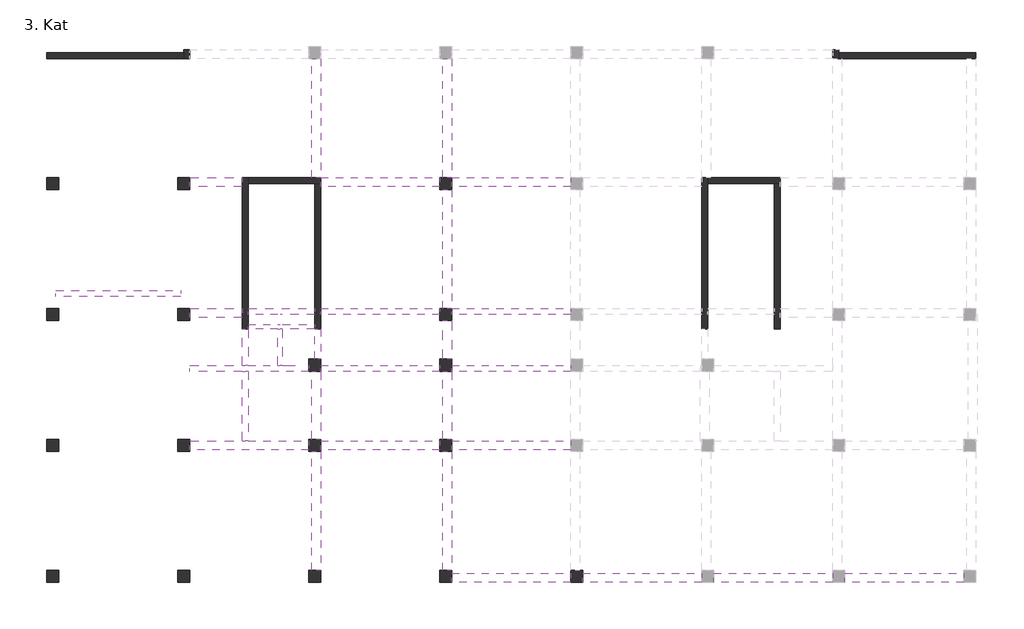
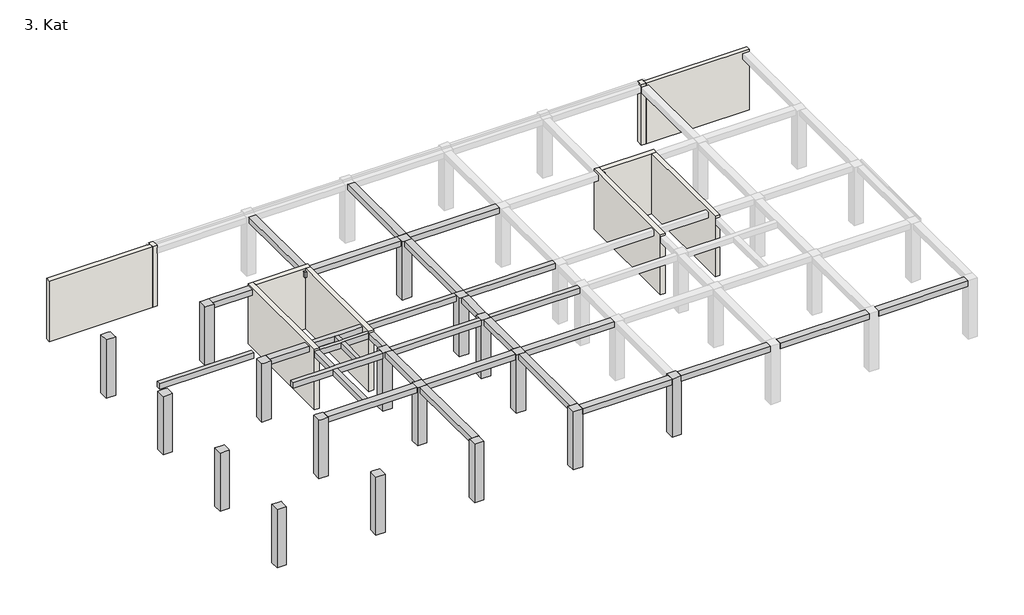
# One storey, part 1 of 2: 31 beams, 17 columns, 10 walls.
"""IFC4 building model written with IfcOpenShell, lengths in millimetres."""

from ifc_helpers import new_model, si_unit, frame, origin, place, context, project, spatial, polyline, outline, extrude, faceted_brep, element, save

model = new_model("IFC4")

# Units and contexts
model_context = context("Model", 3, world=origin())
ifc_project = project(units=[si_unit("LENGTHUNIT", "METRE", prefix="MILLI")], contexts=[model_context])

# Site, building, storey
site = spatial("IfcSite", under=ifc_project)
building = spatial("IfcBuilding", under=site)
storey = spatial("IfcBuildingStorey", under=building, Name="3. Kat", Elevation=15500.0)

# Beams
placement = place(None, origin())
element("IfcBeam", 1, ObjectType="M_Concrete-Rectangular Beam : 40x70cm kiriş 2", at=placement, inside=storey, context=model_context, shape_type="SweptSolid", body=[
    extrude(outline(polyline([(204.0222331, 18150.0006424), (204.0222331, 18550.0006424), (8299.9996735, 18550.0006424), (8299.9996735, 18150.0006424), (204.0222331, 18150.0006424)])), frame((0.0, 0.0, 20300.0), z_axis=(0.0, 0.0, 1.0), x_axis=(1.0, 0.0, 0.0)), (0.0, 0.0, 1.0), 500.0),
])
element("IfcBeam", 2, ObjectType="M_Concrete-Rectangular Beam : 60x70cm kiriş", at=placement, inside=storey, context=model_context, shape_type="SweptSolid", body=[
    extrude(outline(polyline([(16799.9996817, 33600.0009197), (17399.9996817, 33600.0009197), (17399.9996817, 25900.0003816), (16799.9996817, 25900.0003816), (16799.9996817, 33600.0009197)])), frame((0.0, 0.0, 20300.0), z_axis=(0.0, 0.0, 1.0), x_axis=(1.0, 0.0, 0.0)), (0.0, 0.0, 1.0), 500.0),
])
element("IfcBeam", 3, ObjectType="M_Concrete-Rectangular Beam : 60x70cm kiriş", at=placement, inside=storey, context=model_context, shape_type="SweptSolid", body=[
    extrude(outline(polyline([(25899.9996503, 25900.0004105), (25299.9996503, 25900.0004105), (25299.9996503, 33600.0009197), (25899.9996503, 33600.0009197), (25899.9996503, 25900.0004105)])), frame((0.0, 0.0, 20300.0), z_axis=(0.0, 0.0, 1.0), x_axis=(1.0, 0.0, 0.0)), (0.0, 0.0, 1.0), 500.0),
])
element("IfcBeam", 4, ObjectType="M_Concrete-Rectangular Beam : 60x70cm kiriş", at=placement, inside=storey, context=model_context, shape_type="Brep", body=[
    faceted_brep([(25099.9993907, 25900.0000279, 20300.0), (17399.9996817, 25900.0000279, 20300.0), (17399.9996817, 25900.0000279, 20800.0), (25099.9993907, 25900.0000279, 20800.0), (17399.9995362, 25300.0000279, 20300.0), (25099.9993907, 25300.0000279, 20300.0), (25099.9993907, 25300.0000279, 20800.0), (17399.9995362, 25300.0000279, 20800.0)], [[[0, 1, 2, 3]], [[4, 1, 0, 5]], [[5, 6, 7, 4]], [[4, 7, 2, 1]], [[3, 2, 7, 6]], [[5, 0, 3, 6]]]),
    faceted_brep([(16799.9996817, 25500.0003816, 20300.0), (16799.9996817, 25300.0000279, 20300.0), (16799.9996817, 25300.0000279, 20800.0), (16799.9996817, 25500.0003816, 20800.0), (16999.9995362, 25500.0003816, 20800.0), (16999.9995362, 25500.0003816, 20300.0), (16999.9995362, 25300.0000279, 20300.0), (16999.9995362, 25300.0000279, 20800.0)], [[[0, 1, 2, 3]], [[0, 3, 4, 5]], [[6, 5, 4, 7]], [[1, 0, 5, 6]], [[2, 1, 6, 7]], [[3, 2, 7, 4]]]),
])
element("IfcBeam", 5, ObjectType="M_Concrete-Rectangular Beam : 60x70cm kiriş", at=placement, inside=storey, context=model_context, shape_type="SweptSolid", body=[
    extrude(outline(polyline([(8899.9993907, 25299.9999925), (8899.9993907, 25899.9999925), (12300.0064017, 25899.9999925), (12300.0064017, 25299.9999925), (8899.9993907, 25299.9999925)])), frame((0.0, 0.0, 20300.0), z_axis=(0.0, 0.0, 1.0), x_axis=(1.0, 0.0, 0.0)), (0.0, 0.0, 1.0), 500.0),
])
element("IfcBeam", 6, ObjectType="M_Concrete-Rectangular Beam : 60x70cm kiriş", at=placement, inside=storey, context=model_context, shape_type="Brep", body=[
    faceted_brep([(8899.9993907, 16800.0003643, 20800.0), (8899.9993907, 16800.0003643, 20300.0), (12300.0064017, 16800.0003643, 20300.0), (12300.0064017, 16800.0003643, 20800.0), (8899.9996735, 17400.0003643, 20300.0), (12300.0064017, 17400.0003643, 20300.0), (8899.9996735, 17400.0003643, 20800.0), (12300.0064017, 17400.0003643, 20800.0)], [[[0, 1, 2, 3]], [[1, 4, 5, 2]], [[4, 6, 7, 5]], [[6, 4, 1, 0]], [[6, 0, 3, 7]], [[3, 2, 5, 7]]]),
])
element("IfcBeam", 7, ObjectType="M_Concrete-Rectangular Beam : 40x70cm kiriş 2", at=placement, inside=storey, context=model_context, shape_type="Brep", body=[
    faceted_brep([(12700.0064017, 17000.0003638, 20800.0), (12700.0064017, 17000.0003638, 20300.0), (14600.0010318, 17000.0003638, 20300.0), (14900.0010318, 17000.0003638, 20300.0), (16999.9995362, 17000.0003638, 20300.0), (16999.9995362, 17000.0003638, 20800.0), (14900.0010318, 17000.0003638, 20800.0), (14600.0010318, 17000.0003638, 20800.0), (12700.0064017, 17400.0003638, 20300.0), (16999.9995362, 17400.0003638, 20300.0), (12700.0064017, 17400.0003638, 20800.0), (16999.9995362, 17400.0003638, 20800.0)], [[[0, 1, 2, 3, 4, 5, 6, 7]], [[1, 8, 9, 4, 3, 2]], [[8, 10, 11, 9]], [[8, 1, 0, 10]], [[10, 0, 7, 6, 5, 11]], [[5, 4, 9, 11]]]),
])
element("IfcBeam", 8, ObjectType="M_Concrete-Rectangular Beam : 40x70cm kiriş 2", at=placement, inside=storey, context=model_context, shape_type="SweptSolid", body=[
    extrude(outline(polyline([(17399.9995362, 17400.0003766), (25099.999715, 17400.0003766), (25099.999715, 17000.0003766), (17399.9995362, 17000.0003766), (17399.9995362, 17400.0003766)])), frame((0.0, 0.0, 20300.0), z_axis=(0.0, 0.0, 1.0), x_axis=(1.0, 0.0, 0.0)), (0.0, 0.0, 1.0), 500.0),
])
element("IfcBeam", 9, ObjectType="M_Concrete-Rectangular Beam : 40x70cm kiriş 2", at=placement, inside=storey, context=model_context, shape_type="Brep", body=[
    faceted_brep([(16599.9993867, 13700.0003638, 20300.0), (14900.0010318, 13700.0003638, 20300.0), (14600.0010318, 13700.0003638, 20300.0), (12700.0064017, 13700.0003638, 20300.0), (12300.0064017, 13700.0003638, 20300.0), (8899.9996095, 13700.0003638, 20300.0), (8899.9996095, 13700.0003638, 20800.0), (12300.0064017, 13700.0003638, 20800.0), (12700.0064017, 13700.0003638, 20800.0), (14600.0010318, 13700.0003638, 20800.0), (14900.0010318, 13700.0003638, 20800.0), (16599.9993867, 13700.0003638, 20800.0), (16599.9993867, 13300.0003638, 20300.0), (12700.0064017, 13300.0003638, 20300.0), (12300.0064017, 13300.0003638, 20300.0), (8899.9996095, 13300.0003638, 20300.0), (16599.9993867, 13300.0003638, 20800.0), (12700.0064017, 13300.0003638, 20800.0), (12300.0064017, 13300.0003638, 20800.0), (8899.9996095, 13300.0003638, 20800.0)], [[[0, 1, 2, 3, 4, 5, 6, 7, 8, 9, 10, 11]], [[5, 4, 3, 2, 1, 0, 12, 13, 14, 15]], [[15, 14, 13, 12, 16, 17, 18, 19]], [[5, 15, 19, 6]], [[11, 10, 9, 8, 7, 6, 19, 18, 17, 16]], [[12, 0, 11, 16]]]),
])
element("IfcBeam", 10, ObjectType="M_Concrete-Rectangular Beam : 40x70cm kiriş 2", at=placement, inside=storey, context=model_context, shape_type="SweptSolid", body=[
    extrude(outline(polyline([(12700.0064017, 13700.0003638), (12300.0064017, 13700.0003638), (12300.0064017, 16050.000156), (12700.0064017, 16050.000156), (12700.0064017, 13700.0003638)])), frame((0.0, 0.0, 20300.0), z_axis=(0.0, 0.0, 1.0), x_axis=(1.0, 0.0, 0.0)), (0.0, 0.0, 1.0), 500.0),
])
element("IfcBeam", 11, ObjectType="M_Concrete-Rectangular Beam : 40x70cm kiriş 2", at=placement, inside=storey, context=model_context, shape_type="SweptSolid", body=[
    extrude(outline(polyline([(17399.9995362, 14099.9451047), (16999.9995362, 14099.9451047), (16999.9995362, 16050.0003816), (17399.9995362, 16050.0003816), (17399.9995362, 14099.9451047)])), frame((0.0, 0.0, 20300.0), z_axis=(0.0, 0.0, 1.0), x_axis=(1.0, 0.0, 0.0)), (0.0, 0.0, 1.0), 500.0),
])
element("IfcBeam", 12, ObjectType="M_Concrete-Rectangular Beam : 30x70cm kiriş 3", at=placement, inside=storey, context=model_context, shape_type="Brep", body=[
    faceted_brep([(12700.0064017, 16350.0003638, 20300.0), (12700.0064017, 16350.0003638, 20800.0), (14600.0010318, 16350.0003638, 20800.0), (14900.0010318, 16350.0003638, 20800.0), (16999.9995362, 16350.0003638, 20800.0), (16999.9995362, 16350.0003638, 20300.0), (14900.0010318, 16350.0003638, 20300.0), (14600.0010318, 16350.0003638, 20300.0), (16999.9995362, 16050.0003638, 20300.0), (14900.0010318, 16050.0003638, 20300.0), (14600.0010318, 16050.0003638, 20300.0), (12700.0064017, 16050.0003638, 20300.0), (16999.9995362, 16050.0003638, 20800.0), (14900.0010318, 16050.0003638, 20800.0), (14600.0010318, 16050.0003638, 20800.0), (12700.0064017, 16050.0003638, 20800.0)], [[[0, 1, 2, 3, 4, 5, 6, 7]], [[5, 8, 9, 10, 11, 0, 7, 6]], [[11, 10, 9, 8, 12, 13, 14, 15]], [[11, 15, 1, 0]], [[5, 4, 12, 8]], [[15, 14, 13, 12, 4, 3, 2, 1]]]),
])
element("IfcBeam", 13, ObjectType="M_Concrete-Rectangular Beam : 30x70cm kiriş 3", at=placement, inside=storey, context=model_context, shape_type="SweptSolid", body=[
    extrude(outline(polyline([(14900.0010318, 13700.0003638), (14600.0010318, 13700.0003638), (14600.0010318, 16050.0003638), (14900.0010318, 16050.0003638), (14900.0010318, 13700.0003638)])), frame((0.0, 0.0, 20300.0), z_axis=(0.0, 0.0, 1.0), x_axis=(1.0, 0.0, 0.0)), (0.0, 0.0, 1.0), 500.0),
    extrude(outline(polyline([(14600.0010318, 17000.0003638), (14900.0010318, 17000.0003638), (14900.0010318, 16350.0003638), (14600.0010318, 16350.0003638), (14600.0010318, 17000.0003638)])), frame((0.0, 0.0, 20300.0), z_axis=(0.0, 0.0, 1.0), x_axis=(1.0, 0.0, 0.0)), (0.0, 0.0, 1.0), 500.0),
])
element("IfcBeam", 14, ObjectType="M_Concrete-Rectangular Beam : 60x70cm kiriş", at=placement, inside=storey, context=model_context, shape_type="Brep", body=[
    faceted_brep([(8899.9993907, 8200.0009197, 20300.0), (16599.9993907, 8200.0009197, 20300.0), (16599.9993907, 8200.0009197, 20800.0), (8899.9993907, 8200.0009197, 20800.0), (8899.9993907, 8800.0009197, 20300.0), (12300.0064017, 8800.0009197, 20300.0), (12700.0064017, 8800.0009197, 20300.0), (16599.9993907, 8800.0009197, 20300.0), (8899.9993907, 8800.0009197, 20800.0), (12300.0064017, 8800.0009197, 20800.0), (12700.0064017, 8800.0009197, 20800.0), (16599.9993907, 8800.0009197, 20800.0)], [[[0, 1, 2, 3]], [[1, 0, 4, 5, 6, 7]], [[7, 6, 5, 4, 8, 9, 10, 11]], [[3, 2, 11, 10, 9, 8]], [[4, 0, 3, 8]], [[1, 7, 11, 2]]]),
])
element("IfcBeam", 15, ObjectType="M_Concrete-Rectangular Beam : 60x70cm kiriş", at=placement, inside=storey, context=model_context, shape_type="SweptSolid", body=[
    extrude(outline(polyline([(17399.9997293, 8900.0009197), (16799.9997293, 8900.0009197), (16799.9997293, 13299.9451047), (17399.9997293, 13299.9451047), (17399.9997293, 8900.0009197)])), frame((0.0, 0.0, 20300.0), z_axis=(0.0, 0.0, 1.0), x_axis=(1.0, 0.0, 0.0)), (0.0, 0.0, 1.0), 500.0),
])
element("IfcBeam", 16, ObjectType="M_Concrete-Rectangular Beam : 60x70cm kiriş", at=placement, inside=storey, context=model_context, shape_type="SweptSolid", body=[
    extrude(outline(polyline([(16799.9997451, 400.0009197), (16799.9997451, 8099.9999409), (17399.9997451, 8099.9999409), (17399.9997451, 400.0009197), (16799.9997451, 400.0009197)])), frame((0.0, 0.0, 20300.0), z_axis=(0.0, 0.0, 1.0), x_axis=(1.0, 0.0, 0.0)), (0.0, 0.0, 1.0), 500.0),
])
element("IfcBeam", 17, ObjectType="M_Concrete-Rectangular Beam : 40x70cm kiriş 2", at=placement, inside=storey, context=model_context, shape_type="SweptSolid", body=[
    extrude(outline(polyline([(12300.0064017, 13300.0003638), (12700.0064017, 13300.0003638), (12700.0064017, 8800.0009197), (12300.0064017, 8800.0009197), (12300.0064017, 13300.0003638)])), frame((0.0, 0.0, 20300.0), z_axis=(0.0, 0.0, 1.0), x_axis=(1.0, 0.0, 0.0)), (0.0, 0.0, 1.0), 500.0),
])
element("IfcBeam", 18, ObjectType="M_Concrete-Rectangular Beam : 60x70cm kiriş", at=placement, inside=storey, context=model_context, shape_type="SweptSolid", body=[
    extrude(outline(polyline([(25299.9997233, 400.0009197), (25299.9997233, 8100.0009197), (25899.9997233, 8100.0009197), (25899.9997233, 400.0009197), (25299.9997233, 400.0009197)])), frame((0.0, 0.0, 20300.0), z_axis=(0.0, 0.0, 1.0), x_axis=(1.0, 0.0, 0.0)), (0.0, 0.0, 1.0), 500.0),
])
element("IfcBeam", 19, ObjectType="M_Concrete-Rectangular Beam : 60x70cm kiriş", at=placement, inside=storey, context=model_context, shape_type="SweptSolid", body=[
    extrude(outline(polyline([(25099.9993907, 8200.0009197), (17399.9993907, 8200.0009197), (17399.9993907, 8800.0009197), (25099.9993907, 8800.0009197), (25099.9993907, 8200.0009197)])), frame((0.0, 0.0, 20300.0), z_axis=(0.0, 0.0, 1.0), x_axis=(1.0, 0.0, 0.0)), (0.0, 0.0, 1.0), 500.0),
])
element("IfcBeam", 20, ObjectType="M_Concrete-Rectangular Beam : 60x70cm kiriş", at=placement, inside=storey, context=model_context, shape_type="SweptSolid", body=[
    extrude(outline(polyline([(25899.9997233, 8900.0009197), (25299.9997233, 8900.0009197), (25299.9997233, 13300.0003995), (25899.9997233, 13300.0003995), (25899.9997233, 8900.0009197)])), frame((0.0, 0.0, 20300.0), z_axis=(0.0, 0.0, 1.0), x_axis=(1.0, 0.0, 0.0)), (0.0, 0.0, 1.0), 500.0),
])
element("IfcBeam", 21, ObjectType="M_Concrete-Rectangular Beam : 40x70cm kiriş 2", at=placement, inside=storey, context=model_context, shape_type="Brep", body=[
    faceted_brep([(25099.9997415, 13700.0003995, 20800.0), (25099.9997415, 13700.0003995, 20300.0), (17399.9993907, 13700.0003995, 20300.0), (17399.9993907, 13700.0003995, 20800.0), (17399.9997293, 13300.0003995, 20300.0), (25099.9997415, 13300.0003995, 20300.0), (17399.9997293, 13300.0003995, 20800.0), (25099.9997415, 13300.0003995, 20800.0)], [[[0, 1, 2, 3]], [[4, 2, 1, 5]], [[6, 4, 5, 7]], [[4, 6, 3, 2]], [[3, 6, 7, 0]], [[5, 1, 0, 7]]]),
])
element("IfcBeam", 22, ObjectType="M_Concrete-Rectangular Beam : 60x70cm kiriş", at=placement, inside=storey, context=model_context, shape_type="SweptSolid", body=[
    extrude(outline(polyline([(25299.9997233, 14100.0003995), (25299.9997233, 16600.0009197), (25899.9997233, 16600.0009197), (25899.9997233, 14100.0003995), (25299.9997233, 14100.0003995)])), frame((0.0, 0.0, 20300.0), z_axis=(0.0, 0.0, 1.0), x_axis=(1.0, 0.0, 0.0)), (0.0, 0.0, 1.0), 500.0),
])
element("IfcBeam", 23, ObjectType="M_Concrete-Rectangular Beam : 60x70cm kiriş", at=placement, inside=storey, context=model_context, shape_type="SweptSolid", body=[
    extrude(outline(polyline([(25299.999682, 25099.9999518), (25899.999682, 25099.9999518), (25899.999682, 17400.0009197), (25299.999682, 17400.0009197), (25299.999682, 25099.9999518)])), frame((0.0, 0.0, 20300.0), z_axis=(0.0, 0.0, 1.0), x_axis=(1.0, 0.0, 0.0)), (0.0, 0.0, 1.0), 500.0),
])
element("IfcBeam", 24, ObjectType="M_Concrete-Rectangular Beam : 60x70cm kiriş", at=placement, inside=storey, context=model_context, shape_type="Brep", body=[
    faceted_brep([(25899.9996503, 25900.0003995, 20300.0), (25899.9996503, 25900.0003995, 20800.0), (33599.9993907, 25900.0003995, 20800.0), (33599.9993907, 25900.0003995, 20300.0), (25899.9993907, 25300.0003995, 20300.0), (33599.9993907, 25300.0003995, 20300.0), (25899.9993907, 25300.0003995, 20800.0), (33599.9993907, 25300.0003995, 20800.0)], [[[0, 1, 2, 3]], [[4, 0, 3, 5]], [[6, 4, 5, 7]], [[1, 0, 4, 6]], [[1, 6, 7, 2]], [[3, 2, 7, 5]]]),
])
element("IfcBeam", 25, ObjectType="M_Concrete-Rectangular Beam : 40x70cm kiriş 2", at=placement, inside=storey, context=model_context, shape_type="Brep", body=[
    faceted_brep([(33599.9993907, 17000.0007711, 20300.0), (33599.9993907, 17000.0007711, 20800.0), (25899.9993907, 17000.0007711, 20800.0), (25899.9993907, 17000.0007711, 20300.0), (25899.999682, 17400.0007711, 20300.0), (33599.9994953, 17400.0007711, 20300.0), (25899.999682, 17400.0007711, 20800.0), (33599.9994953, 17400.0007711, 20800.0)], [[[0, 1, 2, 3]], [[3, 4, 5, 0]], [[4, 6, 7, 5]], [[3, 2, 6, 4]], [[5, 7, 1, 0]], [[7, 6, 2, 1]]]),
])
element("IfcBeam", 26, ObjectType="M_Concrete-Rectangular Beam : 40x70cm kiriş 2", at=placement, inside=storey, context=model_context, shape_type="Brep", body=[
    faceted_brep([(25899.9997233, 13300.0003995, 20800.0), (25899.9997233, 13300.0003995, 20300.0), (33599.9993907, 13300.0003995, 20300.0), (33599.9993907, 13300.0003995, 20800.0), (25899.9993907, 13700.0003995, 20300.0), (33599.9993907, 13700.0003995, 20300.0), (33599.9993907, 13700.0003995, 20800.0), (25899.9993907, 13700.0003995, 20800.0)], [[[0, 1, 2, 3]], [[1, 4, 5, 2]], [[6, 5, 4, 7]], [[1, 0, 7, 4]], [[7, 0, 3, 6]], [[3, 2, 5, 6]]]),
])
element("IfcBeam", 27, ObjectType="M_Concrete-Rectangular Beam : 60x70cm kiriş", at=placement, inside=storey, context=model_context, shape_type="Brep", body=[
    faceted_brep([(25899.9993907, 8200.0009197, 20800.0), (25899.9993907, 8200.0009197, 20300.0), (33599.9993907, 8200.0009197, 20300.0), (33599.9993907, 8200.0009197, 20800.0), (33599.9994953, 8800.0009197, 20300.0), (25899.9993907, 8800.0009197, 20300.0), (33599.9994953, 8800.0009197, 20800.0), (25899.9993907, 8800.0009197, 20800.0)], [[[0, 1, 2, 3]], [[4, 2, 1, 5]], [[6, 4, 5, 7]], [[4, 6, 3, 2]], [[3, 6, 7, 0]], [[1, 0, 7, 5]]]),
])
element("IfcBeam", 28, ObjectType="M_Concrete-Rectangular Beam : 60x70cm kiriş", at=placement, inside=storey, context=model_context, shape_type="Brep", body=[
    faceted_brep([(34399.9993907, -399.9996882, 20800.0), (34399.9993907, -399.9996882, 20300.0), (42099.9993899, -399.9996882, 20300.0), (42099.9993899, -399.9996882, 20800.0), (42099.999723, 200.0003118, 20300.0), (34399.9993907, 200.0003118, 20300.0), (42099.999723, 200.0003118, 20800.0), (34399.9993907, 200.0003118, 20800.0)], [[[0, 1, 2, 3]], [[4, 2, 1, 5]], [[6, 4, 5, 7]], [[4, 6, 3, 2]], [[3, 6, 7, 0]], [[1, 0, 7, 5]]]),
])
element("IfcBeam", 29, ObjectType="M_Concrete-Rectangular Beam : 60x70cm kiriş", at=placement, inside=storey, context=model_context, shape_type="SweptSolid", body=[
    extrude(outline(polyline([(25899.9993907, -399.9996882), (25899.9993907, 200.0003118), (33599.9993907, 200.0003118), (33599.9993907, -399.9996882), (25899.9993907, -399.9996882)])), frame((0.0, 0.0, 20300.0), z_axis=(0.0, 0.0, 1.0), x_axis=(1.0, 0.0, 0.0)), (0.0, 0.0, 1.0), 500.0),
])
element("IfcBeam", 30, ObjectType="M_Concrete-Rectangular Beam : 60x70cm kiriş", at=placement, inside=storey, context=model_context, shape_type="Brep", body=[
    faceted_brep([(42899.9997771, -399.9996882, 20800.0), (42899.9997771, -399.9996882, 20300.0), (50599.9993899, -399.9996882, 20300.0), (50599.9993899, -399.9996882, 20800.0), (50599.999723, 200.0003118, 20300.0), (42899.9997771, 200.0003118, 20300.0), (50599.999723, 200.0003118, 20800.0), (42899.9997771, 200.0003118, 20800.0)], [[[0, 1, 2, 3]], [[4, 2, 1, 5]], [[6, 4, 5, 7]], [[4, 6, 3, 2]], [[3, 6, 7, 0]], [[5, 1, 0, 7]]]),
])
element("IfcBeam", 31, ObjectType="M_Concrete-Rectangular Beam : 60x70cm kiriş", at=placement, inside=storey, context=model_context, shape_type="SweptSolid", body=[
    extrude(outline(polyline([(59099.9997769, -399.9996882), (51399.9997769, -399.9996882), (51399.9997769, 200.0003118), (59099.9997769, 200.0003118), (59099.9997769, -399.9996882)])), frame((0.0, 0.0, 20300.0), z_axis=(0.0, 0.0, 1.0), x_axis=(1.0, 0.0, 0.0)), (0.0, 0.0, 1.0), 500.0),
])

# Columns
element("IfcColumn", 32, ObjectType="M_Concrete-Rectangular-Column : 80x80cm kolon", at=placement, inside=storey, context=model_context, shape_type="Brep", body=[
    faceted_brep([(400.0000836, 400.0009197, 15500.0), (400.0000836, -399.9990803, 15500.0), (-399.9999164, -399.9990803, 15500.0), (-399.9999164, 400.0009197, 15500.0), (400.0000836, 400.0009197, 20800.0), (400.0000836, 199.9995192, 20800.0), (400.0000836, -399.9990803, 20800.0), (-399.9999164, -399.9990803, 20800.0), (-399.9999164, 400.0009197, 20800.0), (199.9996111, 400.0009197, 20800.0)], [[[0, 1, 2, 3]], [[1, 0, 4, 5, 6]], [[2, 1, 6, 7]], [[3, 2, 7, 8]], [[0, 3, 8, 9, 4]], [[6, 5, 4, 9, 8, 7]]]),
])
element("IfcColumn", 33, ObjectType="M_Concrete-Rectangular-Column : 80x80cm kolon", at=placement, inside=storey, context=model_context, shape_type="Brep", body=[
    faceted_brep([(8899.9993907, 400.0009197, 15500.0), (8899.9993907, -399.9990803, 15500.0), (8099.9993907, -399.9990803, 15500.0), (8099.9993907, 400.0009197, 15500.0), (8899.9993907, 400.0009197, 20800.0), (8899.9993907, 199.9999577, 20800.0), (8899.9993907, -399.9990803, 20800.0), (8099.9993907, -399.9990803, 20800.0), (8099.9993907, 199.9995192, 20800.0), (8099.9993907, 400.0009197, 20800.0), (8299.9996095, 400.0009197, 20800.0)], [[[0, 1, 2, 3]], [[1, 0, 4, 5, 6]], [[2, 1, 6, 7]], [[3, 2, 7, 8, 9]], [[0, 3, 9, 10, 4]], [[6, 5, 4, 10, 9, 8, 7]]]),
])
element("IfcColumn", 34, ObjectType="M_Concrete-Rectangular-Column : 80x80cm kolon", at=placement, inside=storey, context=model_context, shape_type="Brep", body=[
    faceted_brep([(400.0000836, 8900.0009197, 15500.0), (400.0000836, 8100.0009197, 15500.0), (-399.9999164, 8100.0009197, 15500.0), (-399.9999164, 8900.0009197, 15500.0), (400.0000836, 8900.0009197, 20800.0), (400.0000836, 8800.0009197, 20800.0), (400.0000836, 8200.0009197, 20800.0), (400.0000836, 8100.0009197, 20800.0), (199.9996111, 8100.0009197, 20800.0), (-399.9999164, 8100.0009197, 20800.0), (-399.9999164, 8900.0009197, 20800.0), (199.9996411, 8900.0009197, 20800.0)], [[[0, 1, 2, 3]], [[1, 0, 4, 5, 6, 7]], [[2, 1, 7, 8, 9]], [[3, 2, 9, 10]], [[0, 3, 10, 11, 4]], [[7, 6, 5, 4, 11, 10, 9, 8]]]),
])
element("IfcColumn", 35, ObjectType="M_Concrete-Rectangular-Column : 80x80cm kolon", at=placement, inside=storey, context=model_context, shape_type="Brep", body=[
    faceted_brep([(8899.9993907, 8900.0009197, 15500.0), (8899.9993907, 8100.0009197, 15500.0), (8099.9993907, 8100.0009197, 15500.0), (8099.9993907, 8900.0009197, 15500.0), (8899.9993907, 8900.0009197, 20800.0), (8899.9993907, 8800.0009197, 20800.0), (8899.9993907, 8200.0009197, 20800.0), (8899.9993907, 8100.0009197, 20800.0), (8299.9996095, 8100.0009197, 20800.0), (8099.9993907, 8100.0009197, 20800.0), (8099.9993907, 8200.0009197, 20800.0), (8099.9993907, 8800.0009197, 20800.0), (8099.9993907, 8900.0009197, 20800.0), (8299.9996095, 8900.0009197, 20800.0)], [[[0, 1, 2, 3]], [[1, 0, 4, 5, 6, 7]], [[2, 1, 7, 8, 9]], [[3, 2, 9, 10, 11, 12]], [[0, 3, 12, 13, 4]], [[7, 6, 5, 4, 13, 12, 11, 10, 9, 8]]]),
])
element("IfcColumn", 36, ObjectType="M_Concrete-Rectangular-Column : 80x80cm kolon", at=placement, inside=storey, context=model_context, shape_type="Brep", body=[
    faceted_brep([(8899.9993907, 17400.0009197, 15500.0), (8899.9993907, 16600.0009197, 15500.0), (8099.9993907, 16600.0009197, 15500.0), (8099.9993907, 17400.0009197, 15500.0), (8899.9993907, 17400.0009197, 20800.0), (8899.9993907, 16800.0003643, 20800.0), (8899.9993907, 16600.0009197, 20800.0), (8299.9996095, 16600.0009197, 20800.0), (8099.9993907, 16600.0009197, 20800.0), (8099.9993907, 16800.0003638, 20800.0), (8099.9993907, 17400.0009197, 20800.0), (8299.9996735, 17400.0009197, 20800.0)], [[[0, 1, 2, 3]], [[1, 0, 4, 5, 6]], [[2, 1, 6, 7, 8]], [[3, 2, 8, 9, 10]], [[0, 3, 10, 11, 4]], [[6, 5, 4, 11, 10, 9, 8, 7]]]),
])
element("IfcColumn", 37, ObjectType="M_Concrete-Rectangular-Column : 80x80cm kolon", at=placement, inside=storey, context=model_context, shape_type="Brep", body=[
    faceted_brep([(400.0000836, 17400.0009197, 15500.0), (400.0000836, 16600.0009197, 15500.0), (-399.9999164, 16600.0009197, 15500.0), (-399.9999164, 17400.0009197, 15500.0), (400.0000836, 17400.0009197, 20800.0), (400.0000836, 16800.0003638, 20800.0), (400.0000836, 16600.0009197, 20800.0), (199.9996411, 16600.0009197, 20800.0), (-399.9999164, 16600.0009197, 20800.0), (-399.9999164, 17400.0009197, 20800.0), (199.9994072, 17400.0009197, 20800.0)], [[[0, 1, 2, 3]], [[1, 0, 4, 5, 6]], [[2, 1, 6, 7, 8]], [[3, 2, 8, 9]], [[0, 3, 9, 10, 4]], [[6, 5, 4, 10, 9, 8, 7]]]),
])
element("IfcColumn", 38, ObjectType="M_Concrete-Rectangular-Column : 80x80cm kolon", at=placement, inside=storey, context=model_context, shape_type="Brep", body=[
    faceted_brep([(399.9996699, 25899.9999188, 15500.0), (399.9996699, 25099.9999188, 15500.0), (-400.0003301, 25099.9999188, 15500.0), (-400.0003301, 25899.9999188, 15500.0), (399.9996699, 25899.9999188, 20800.0), (399.9996699, 25299.999992, 20800.0), (399.9996699, 25099.9999188, 20800.0), (199.9994072, 25099.9999188, 20800.0), (-400.0003301, 25099.9999188, 20800.0), (-400.0003301, 25899.9999188, 20800.0), (199.9994681, 25899.9999188, 20800.0)], [[[0, 1, 2, 3]], [[1, 0, 4, 5, 6]], [[2, 1, 6, 7, 8]], [[3, 2, 8, 9]], [[0, 3, 9, 10, 4]], [[6, 5, 4, 10, 9, 8, 7]]]),
])
element("IfcColumn", 39, ObjectType="M_Concrete-Rectangular-Column : 80x80cm kolon", at=placement, inside=storey, context=model_context, shape_type="Brep", body=[
    faceted_brep([(8899.9993907, 25899.9999188, 15500.0), (8899.9993907, 25099.9999188, 15500.0), (8099.9993907, 25099.9999188, 15500.0), (8099.9993907, 25899.9999188, 15500.0), (8899.9993907, 25899.9999188, 20300.0), (8899.9993907, 25899.9999188, 20800.0), (8899.9993907, 25299.9999925, 20800.0), (8899.9993907, 25099.9999188, 20800.0), (8299.9996735, 25099.9999188, 20800.0), (8099.9993907, 25099.9999188, 20800.0), (8099.9993907, 25299.999992, 20800.0), (8099.9993907, 25899.9999188, 20800.0), (8299.9993907, 25899.9999188, 20800.0)], [[[0, 1, 2, 3]], [[1, 0, 4, 5, 6, 7]], [[2, 1, 7, 8, 9]], [[3, 2, 9, 10, 11]], [[0, 3, 11, 12, 5, 4]], [[7, 6, 5, 12, 11, 10, 9, 8]]]),
])
element("IfcColumn", 40, ObjectType="M_Concrete-Rectangular-Column : 80x80cm kolon", at=placement, inside=storey, context=model_context, shape_type="Brep", body=[
    faceted_brep([(17399.9993907, 8900.0009197, 15500.0), (17399.9993907, 8100.0009197, 15500.0), (16599.9993907, 8100.0009197, 15500.0), (16599.9993907, 8900.0009197, 15500.0), (17399.9993907, 8900.0009197, 20800.0), (17399.9993907, 8800.0009197, 20800.0), (17399.9993907, 8200.0009197, 20800.0), (17399.9993907, 8100.0009197, 20800.0), (16799.9997451, 8100.0009197, 20800.0), (16599.9993907, 8100.0009197, 20800.0), (16599.9993907, 8200.0009197, 20800.0), (16599.9993907, 8800.0009197, 20800.0), (16599.9993907, 8900.0009197, 20800.0), (16799.9997293, 8900.0009197, 20800.0)], [[[0, 1, 2, 3]], [[1, 0, 4, 5, 6, 7]], [[2, 1, 7, 8, 9]], [[3, 2, 9, 10, 11, 12]], [[0, 3, 12, 13, 4]], [[7, 6, 5, 4, 13, 12, 11, 10, 9, 8]]]),
])
element("IfcColumn", 41, ObjectType="M_Concrete-Rectangular-Column : 80x80cm kolon", at=placement, inside=storey, context=model_context, shape_type="Brep", body=[
    faceted_brep([(25899.9993907, 8900.0009197, 15500.0), (25899.9993907, 8100.0009197, 15500.0), (25099.9993907, 8100.0009197, 15500.0), (25099.9993907, 8900.0009197, 15500.0), (25899.9993907, 8900.0009197, 20800.0), (25899.9993907, 8800.0009197, 20800.0), (25899.9993907, 8200.0009197, 20800.0), (25899.9993907, 8100.0009197, 20800.0), (25299.9997233, 8100.0009197, 20800.0), (25099.9993907, 8100.0009197, 20800.0), (25099.9993907, 8200.0009197, 20800.0), (25099.9993907, 8800.0009197, 20800.0), (25099.9993907, 8900.0009197, 20800.0), (25299.9997233, 8900.0009197, 20800.0)], [[[0, 1, 2, 3]], [[1, 0, 4, 5, 6, 7]], [[2, 1, 7, 8, 9]], [[3, 2, 9, 10, 11, 12]], [[0, 3, 12, 13, 4]], [[7, 6, 5, 4, 13, 12, 11, 10, 9, 8]]]),
])
element("IfcColumn", 42, ObjectType="M_Concrete-Rectangular-Column : 80x80cm kolon", at=placement, inside=storey, context=model_context, shape_type="Brep", body=[
    faceted_brep([(25899.9993907, 400.0009197, 15500.0), (25899.9993907, -399.9990803, 15500.0), (25099.9993907, -399.9990803, 15500.0), (25099.9993907, 400.0009197, 15500.0), (25899.9993907, 400.0009197, 20800.0), (25899.9993907, 200.0003118, 20800.0), (25899.9993907, -399.9990803, 20800.0), (25099.9993907, -399.9990803, 20800.0), (25099.9993907, 200.0003837, 20800.0), (25099.9993907, 400.0009197, 20800.0), (25299.9997233, 400.0009197, 20800.0)], [[[0, 1, 2, 3]], [[1, 0, 4, 5, 6]], [[2, 1, 6, 7]], [[3, 2, 7, 8, 9]], [[0, 3, 9, 10, 4]], [[6, 5, 4, 10, 9, 8, 7]]]),
])
element("IfcColumn", 43, ObjectType="M_Concrete-Rectangular-Column : 80x80cm kolon", at=placement, inside=storey, context=model_context, shape_type="Brep", body=[
    faceted_brep([(17399.9993907, 400.0009197, 15500.0), (17399.9993907, -399.9990803, 15500.0), (16599.9993907, -399.9990803, 15500.0), (16599.9993907, 400.0009197, 15500.0), (17399.9993907, 400.0009197, 20800.0), (17399.9993907, 200.0003837, 20800.0), (17399.9993907, -399.9990803, 20800.0), (16599.9993907, -399.9990803, 20800.0), (16599.9993907, 199.9999577, 20800.0), (16599.9993907, 400.0009197, 20800.0), (16799.9997451, 400.0009197, 20800.0)], [[[0, 1, 2, 3]], [[1, 0, 4, 5, 6]], [[2, 1, 6, 7]], [[3, 2, 7, 8, 9]], [[0, 3, 9, 10, 4]], [[6, 5, 4, 10, 9, 8, 7]]]),
])
element("IfcColumn", 44, ObjectType="M_Concrete-Rectangular-Column : 80x80cm kolon", at=placement, inside=storey, context=model_context, shape_type="Brep", body=[
    faceted_brep([(34399.9993907, 400.0009197, 15500.0), (34399.9993907, -399.9990803, 15500.0), (33599.9993907, -399.9990803, 15500.0), (33599.9993907, 400.0009197, 15500.0), (34399.9993907, 400.0009197, 20800.0), (34399.9993907, 200.0003118, 20800.0), (34399.9993907, -399.9990803, 20800.0), (33599.9993907, -399.9990803, 20800.0), (33599.9993907, 200.0003118, 20800.0), (33599.9993907, 400.0009197, 20800.0), (34199.9997451, 400.0009197, 20800.0)], [[[0, 1, 2, 3]], [[1, 0, 4, 5, 6]], [[2, 1, 6, 7]], [[3, 2, 7, 8, 9]], [[0, 3, 9, 10, 4]], [[6, 5, 4, 10, 9, 8, 7]]]),
])
element("IfcColumn", 45, ObjectType="M_Concrete-Rectangular-Column : 80x80cm kolon", at=placement, inside=storey, context=model_context, shape_type="Brep", body=[
    faceted_brep([(25899.9993907, 17400.0009197, 15500.0), (25899.9993907, 16600.0009197, 15500.0), (25099.9993907, 16600.0009197, 15500.0), (25099.9993907, 17400.0009197, 15500.0), (25899.9993907, 17400.0009197, 20800.0), (25899.9993907, 17000.0007711, 20800.0), (25899.9993907, 16600.0009197, 20800.0), (25299.9997233, 16600.0009197, 20800.0), (25099.9993907, 16600.0009197, 20800.0), (25099.9993907, 17000.0003766, 20800.0), (25099.9993907, 17400.0009197, 20800.0), (25299.999682, 17400.0009197, 20800.0)], [[[0, 1, 2, 3]], [[1, 0, 4, 5, 6]], [[2, 1, 6, 7, 8]], [[3, 2, 8, 9, 10]], [[0, 3, 10, 11, 4]], [[6, 5, 4, 11, 10, 9, 8, 7]]]),
])
element("IfcColumn", 46, ObjectType="M_Concrete-Rectangular-Column : 80x80cm kolon", at=placement, inside=storey, context=model_context, shape_type="Brep", body=[
    faceted_brep([(25899.9993907, 14100.0003995, 15500.0), (25899.9993907, 13300.0003995, 15500.0), (25099.9993907, 13300.0003995, 15500.0), (25099.9993907, 14100.0003995, 15500.0), (25899.9993907, 14100.0003995, 20800.0), (25899.9993907, 13700.0003995, 20800.0), (25899.9993907, 13300.0003995, 20800.0), (25899.9993907, 13300.0003995, 20300.0), (25299.9997233, 13300.0003995, 20800.0), (25099.9993907, 13300.0003995, 20800.0), (25099.9993907, 13300.0003995, 20300.0), (25099.9993907, 13700.0003995, 20800.0), (25099.9993907, 14100.0003995, 20800.0), (25299.9997233, 14100.0003995, 20800.0)], [[[0, 1, 2, 3]], [[1, 0, 4, 5, 6, 7]], [[2, 1, 7, 6, 8, 9, 10]], [[3, 2, 10, 9, 11, 12]], [[0, 3, 12, 13, 4]], [[6, 5, 4, 13, 12, 11, 9, 8]]]),
])
element("IfcColumn", 47, ObjectType="M_Concrete-Rectangular-Column : 80x80cm kolon", at=placement, inside=storey, context=model_context, shape_type="Brep", body=[
    faceted_brep([(17399.9993907, 14099.9451047, 15500.0), (17399.9993907, 13299.9451047, 15500.0), (16599.9993907, 13299.9451047, 15500.0), (16599.9993907, 14099.9451047, 15500.0), (17399.9993907, 14099.9451047, 20800.0), (17399.9993907, 13700.0003995, 20800.0), (17399.9993907, 13299.9451047, 20800.0), (16799.9997293, 13299.9451047, 20800.0), (16599.9993907, 13299.9451047, 20800.0), (16599.9993907, 13700.0003638, 20800.0), (16599.9993907, 14099.9451047, 20800.0), (16999.9995362, 14099.9451047, 20800.0)], [[[0, 1, 2, 3]], [[1, 0, 4, 5, 6]], [[2, 1, 6, 7, 8]], [[3, 2, 8, 9, 10]], [[0, 3, 10, 11, 4]], [[6, 5, 4, 11, 10, 9, 8, 7]]]),
])
element("IfcColumn", 48, ObjectType="M_Concrete-Rectangular-Column : 80x80cm kolon", at=placement, inside=storey, context=model_context, shape_type="Brep", body=[
    faceted_brep([(25899.9993907, 25900.0004105, 15500.0), (25899.9993907, 25100.0004105, 15500.0), (25099.9993907, 25100.0004105, 15500.0), (25099.9993907, 25900.0004105, 15500.0), (25899.9993907, 25900.0004105, 20800.0), (25899.9993907, 25300.0003995, 20800.0), (25899.9993907, 25100.0004105, 20800.0), (25299.999682, 25100.0004105, 20800.0), (25099.9993907, 25100.0004105, 20800.0), (25099.9993907, 25300.0000279, 20800.0), (25099.9993907, 25900.0004105, 20800.0), (25299.9996503, 25900.0004105, 20800.0)], [[[0, 1, 2, 3]], [[1, 0, 4, 5, 6]], [[2, 1, 6, 7, 8]], [[3, 2, 8, 9, 10]], [[0, 3, 10, 11, 4]], [[6, 5, 4, 11, 10, 9, 8, 7]]]),
])

# Walls
element("IfcWall", 49, ObjectType="40cm perde duvar", at=placement, inside=storey, context=model_context, shape_type="Brep", body=[
    faceted_brep([(-400.0005319, 33600.0004302, 15500.0), (8499.9995273, 33600.0004302, 15500.0), (8499.9995273, 33600.0004302, 21000.0), (-400.0005319, 33600.0004302, 21000.0), (-400.0005319, 33600.0004302, 20800.0), (-400.0005319, 33600.0004302, 20300.0), (-400.0005319, 34000.0004302, 15500.0), (-400.0005319, 34000.0004302, 21000.0), (8299.9993907, 34000.0004302, 21000.0), (8499.9995273, 34000.0004302, 21000.0), (8499.9995273, 34000.0004302, 20300.0), (8499.9995273, 34000.0004302, 15500.0)], [[[0, 1, 2, 3, 4, 5]], [[6, 7, 8, 9, 10, 11]], [[1, 0, 6, 11]], [[3, 2, 9, 8, 7]], [[0, 5, 4, 3, 7, 6]], [[2, 1, 11, 10, 9]]]),
])
element("IfcWall", 50, ObjectType="40cm perde duvar", at=placement, inside=storey, context=model_context, shape_type="Brep", body=[
    faceted_brep([(8899.9995273, 33600.0004302, 15500.0), (8899.9995273, 34200.0004302, 15500.0), (8899.9995273, 34200.0004302, 21000.0), (8899.9995273, 34000.0004302, 21000.0), (8899.9995273, 33600.0004302, 21000.0), (8499.9995273, 33600.0004302, 15500.0), (8499.9995273, 33600.0004302, 21000.0), (8499.9995273, 34000.0004302, 21000.0), (8499.9995273, 34200.0004302, 21000.0), (8499.9995273, 34200.0004302, 15500.0), (8499.9995273, 34000.0004302, 15500.0)], [[[0, 1, 2, 3, 4]], [[5, 6, 7, 8, 9, 10]], [[1, 0, 5, 10, 9]], [[2, 1, 9, 8]], [[4, 3, 2, 8, 7, 6]], [[0, 4, 6, 5]]]),
])
element("IfcWall", 51, ObjectType="40cm perde duvar", at=placement, inside=storey, context=model_context, shape_type="Brep", body=[
    faceted_brep([(12700.0064017, 16050.000156, 15500.0), (12700.0064017, 25500.0003816, 15500.0), (12700.0064017, 25900.0003816, 15500.0), (12700.0064017, 25900.0003816, 21000.0), (12700.0064017, 25500.0003816, 21000.0), (12700.0064017, 16050.000156, 21000.0), (12700.0064017, 16050.000156, 20800.0), (12700.0064017, 16050.000156, 20300.0), (12300.0064017, 16050.000156, 15500.0), (12300.0064017, 16050.000156, 20300.0), (12300.0064017, 16050.000156, 20800.0), (12300.0064017, 16050.000156, 21000.0), (12300.0064017, 25900.0003816, 21000.0), (12300.0064017, 25900.0003816, 15500.0)], [[[0, 1, 2, 3, 4, 5, 6, 7]], [[8, 9, 10, 11, 12, 13]], [[2, 1, 0, 8, 13]], [[5, 4, 3, 12, 11]], [[0, 7, 6, 5, 11, 10, 9, 8]], [[3, 2, 13, 12]]]),
])
element("IfcWall", 52, ObjectType="40cm perde duvar", at=placement, inside=storey, context=model_context, shape_type="Brep", body=[
    faceted_brep([(12700.0064017, 25500.0003816, 15500.0), (16999.9995362, 25500.0003816, 15500.0), (17399.9995362, 25500.0003816, 15500.0), (17399.9995362, 25500.0003816, 21000.0), (16999.9995362, 25500.0003816, 21000.0), (12700.0064017, 25500.0003816, 21000.0), (12700.0064017, 25900.0003816, 15500.0), (12700.0064017, 25900.0003816, 21000.0), (17399.9995362, 25900.0003816, 21000.0), (17399.9995362, 25900.0003816, 15500.0)], [[[0, 1, 2, 3, 4, 5]], [[6, 7, 8, 9]], [[2, 1, 0, 6, 9]], [[5, 4, 3, 8, 7]], [[0, 5, 7, 6]], [[3, 2, 9, 8]]]),
])
element("IfcWall", 53, ObjectType="40cm perde duvar", at=placement, inside=storey, context=model_context, shape_type="Brep", body=[
    faceted_brep([(16999.9995362, 25500.0003816, 15500.0), (16999.9995362, 16050.0003816, 15500.0), (16999.9995362, 16050.0003816, 20300.0), (16999.9995362, 16050.0003816, 20800.0), (16999.9995362, 16050.0003816, 21000.0), (16999.9995362, 25500.0003816, 21000.0), (16999.9995362, 25500.0003816, 20800.0), (16999.9995362, 25500.0003816, 20300.0), (17399.9995362, 25500.0003816, 15500.0), (17399.9995362, 25500.0003816, 21000.0), (17399.9995362, 16050.0003816, 21000.0), (17399.9995362, 16050.0003816, 20800.0), (17399.9995362, 16050.0003816, 20300.0), (17399.9995362, 16050.0003816, 15500.0)], [[[0, 1, 2, 3, 4, 5, 6, 7]], [[8, 9, 10, 11, 12, 13]], [[1, 0, 8, 13]], [[4, 3, 2, 1, 13, 12, 11, 10]], [[5, 4, 10, 9]], [[0, 7, 6, 5, 9, 8]]]),
])
element("IfcWall", 54, ObjectType="40cm perde duvar", at=placement, inside=storey, context=model_context, shape_type="Brep", body=[
    faceted_brep([(42499.9995162, 16050.0004138, 15500.0), (42499.9995162, 25500.0004459, 15500.0), (42499.9995162, 25900.0004459, 15500.0), (42499.9995162, 25900.0004459, 21000.0), (42499.9995162, 25500.0004459, 21000.0), (42499.9995162, 16050.0004138, 21000.0), (42499.9995162, 16050.0004138, 20800.0), (42499.9995162, 16050.0004138, 20300.0), (42099.9995162, 16050.0004138, 15500.0), (42099.9995162, 16050.0004138, 20300.0), (42099.9995162, 16050.0004138, 20800.0), (42099.9995162, 16050.0004138, 21000.0), (42099.9995162, 25900.0004459, 21000.0), (42099.9995162, 25900.0004459, 15500.0)], [[[0, 1, 2, 3, 4, 5, 6, 7]], [[8, 9, 10, 11, 12, 13]], [[2, 1, 0, 8, 13]], [[5, 4, 3, 12, 11]], [[0, 7, 6, 5, 11, 10, 9, 8]], [[3, 2, 13, 12]]]),
])
element("IfcWall", 55, ObjectType="40cm perde duvar", at=placement, inside=storey, context=model_context, shape_type="Brep", body=[
    faceted_brep([(42499.9995162, 25500.0004459, 15500.0), (46799.999381, 25500.0004459, 15500.0), (47199.999381, 25500.0004459, 15500.0), (47199.999381, 25500.0004459, 21000.0), (46799.999381, 25500.0004459, 21000.0), (42499.9995162, 25500.0004459, 21000.0), (42499.9995162, 25500.0004459, 20800.0), (42499.9995162, 25500.0004459, 20300.0), (42499.9995162, 25900.0004459, 15500.0), (42499.9995162, 25900.0004459, 21000.0), (47199.999381, 25900.0004459, 21000.0), (47199.999381, 25900.0004459, 15500.0)], [[[0, 1, 2, 3, 4, 5, 6, 7]], [[8, 9, 10, 11]], [[2, 1, 0, 8, 11]], [[5, 4, 3, 10, 9]], [[0, 7, 6, 5, 9, 8]], [[3, 2, 11, 10]]]),
])
element("IfcWall", 56, ObjectType="40cm perde duvar", at=placement, inside=storey, context=model_context, shape_type="Brep", body=[
    faceted_brep([(46799.999381, 25500.0004459, 15500.0), (46799.999381, 16050.0004138, 15500.0), (46799.999381, 16050.0004138, 20300.0), (46799.999381, 16050.0004138, 20800.0), (46799.999381, 16050.0004138, 21000.0), (46799.999381, 25500.0004459, 21000.0), (47199.999381, 25500.0004459, 15500.0), (47199.999381, 25500.0004459, 21000.0), (47199.999381, 16050.0004138, 21000.0), (47199.999381, 16050.0004138, 20800.0), (47199.999381, 16050.0004138, 20300.0), (47199.999381, 16050.0004138, 15500.0)], [[[0, 1, 2, 3, 4, 5]], [[6, 7, 8, 9, 10, 11]], [[1, 0, 6, 11]], [[4, 3, 2, 1, 11, 10, 9, 8]], [[5, 4, 8, 7]], [[0, 5, 7, 6]]]),
])
element("IfcWall", 57, ObjectType="40cm perde duvar", at=placement, inside=storey, context=model_context, shape_type="Brep", body=[
    faceted_brep([(50599.9994944, 34193.7257565, 15500.0), (50599.9994944, 33600.0004303, 15500.0), (50599.9994944, 33600.0004303, 21000.0), (50599.9994944, 34000.0004302, 21000.0), (50599.9994944, 34193.7257565, 21000.0), (50599.9994944, 34193.7257565, 20300.0), (50999.9994944, 34193.7257565, 15500.0), (50999.9994944, 34193.7257565, 20300.0), (50999.9994944, 34193.7257565, 21000.0), (50999.9994944, 34000.0004303, 21000.0), (50999.9994944, 33600.0004303, 21000.0), (50999.9994944, 33600.0004303, 15500.0), (50999.9994944, 34000.0004303, 15500.0)], [[[0, 1, 2, 3, 4, 5]], [[6, 7, 8, 9, 10, 11, 12]], [[1, 0, 6, 12, 11]], [[4, 3, 2, 10, 9, 8]], [[0, 5, 4, 8, 7, 6]], [[2, 1, 11, 10]]]),
])
element("IfcWall", 58, ObjectType="40cm perde duvar", at=placement, inside=storey, context=model_context, shape_type="Brep", body=[
    faceted_brep([(50999.9994944, 33600.0004303, 15500.0), (59899.9999497, 33600.0004303, 15500.0), (59899.9999497, 33600.0004303, 21000.0), (50999.9994944, 33600.0004303, 21000.0), (50999.9994944, 34000.0004303, 15500.0), (50999.9994944, 34000.0004303, 20300.0), (50999.9994944, 34000.0004303, 21000.0), (51199.9994348, 34000.0004303, 21000.0), (59899.9999497, 34000.0004303, 21000.0), (59899.9999497, 34000.0004303, 15500.0)], [[[0, 1, 2, 3]], [[4, 5, 6, 7, 8, 9]], [[1, 0, 4, 9]], [[2, 1, 9, 8]], [[3, 2, 8, 7, 6]], [[0, 3, 6, 5, 4]]]),
])

save(model, "model.ifc")

# Revit data of these elements
# Project information
#   Project Issue Date = "Issue Date"
#   Project Status = "Project Status"
#   Client Name = "Owner"
#   Project Address = "Enter address here"
#   Project Name = "Project Name"
#   Project Number = "0001"
# Type "M_Concrete-Rectangular Beam : 40x70cm kiriş 2"
#   Length [instance default] = 152.4 cm
#   b = 40 cm
#   h = 70 cm
#   Structural Material [instance default] = Concrete, Cast-in-Place gray
#   Assembly Code = ""
# Type "M_Concrete-Rectangular Beam : 60x70cm kiriş"
#   Length [instance default] = 152.4 cm
#   b = 60 cm
#   h = 70 cm
#   Structural Material [instance default] = Concrete, Cast-in-Place gray
#   Assembly Code = ""
# Type "M_Concrete-Rectangular Beam : 30x70cm kiriş 3"
#   Length [instance default] = 152.4 cm
#   b = 30 cm
#   h = 70 cm
#   Structural Material [instance default] = Concrete, Cast-in-Place gray
#   Assembly Code = ""
# Type "M_Concrete-Rectangular-Column : 80x80cm kolon"
#   b = 80 cm
#   h = 80 cm
#   Structural Material [instance default] = Concrete, Cast-in-Place gray
# Type "40cm perde duvar"
#   Layers, outside or top first: 40 cm no material (function 1)
# Elements 1, 7, 8, 9, 10, 11, 17, 21, 25, 26 (IfcBeam, "M_Concrete-Rectangular Beam : 40x70cm kiriş 2")
#   Comments = ""
#   Structural Material = Concrete, Cast-in-Place gray
#   Phase Created = New Construction
#   Materials on its faces: "Concrete, Cast-in-Place gray"
# Elements 2, 3, 4, 5, 6, 14, 15, 16, 18, 19, 20, 22, 23, 24, 27, 28, 29, 30, 31 (IfcBeam, "M_Concrete-Rectangular Beam : 60x70cm kiriş")
#   Comments = ""
#   Structural Material = Concrete, Cast-in-Place gray
#   Phase Created = New Construction
#   Materials on its faces: "Concrete, Cast-in-Place gray"
# Elements 12, 13 (IfcBeam, "M_Concrete-Rectangular Beam : 30x70cm kiriş 3")
#   Comments = ""
#   Structural Material = Concrete, Cast-in-Place gray
#   Phase Created = New Construction
#   Materials on its faces: "Concrete, Cast-in-Place gray"
# Elements 32, 33, 34, 35, 36, 37, 38, 39, 40, 41, 42, 43, 44, 45, 46, 47, 48 (IfcColumn, "M_Concrete-Rectangular-Column : 80x80cm kolon")
#   Structural Material = Concrete, Cast-in-Place gray
#   Phase Created = New Construction
#   Materials on its faces: "Concrete, Cast-in-Place gray"
# Elements 49, 50, 51, 52, 53, 54, 55, 56, 57, 58 (IfcWall, "40cm perde duvar")
#   Comments = ""
#   Top Offset = 0 cm
#   Base Offset = 0 cm
#   wall height = 550 cm
#   Phase Created = New Construction
#   Base Constraint = 3. Kat
#   Top Constraint = 4. Kat
#   Materials on its faces: "Default Wall"
# Materials
#   "Concrete, Cast-in-Place gray": class "Concrete", colour RGB 192 192 192, transparency 0, Description = "Cast-in-place concrete", Cost = 0
#   "Default Wall": class "Miscellaneous", colour RGB 128 128 128, transparency 0
